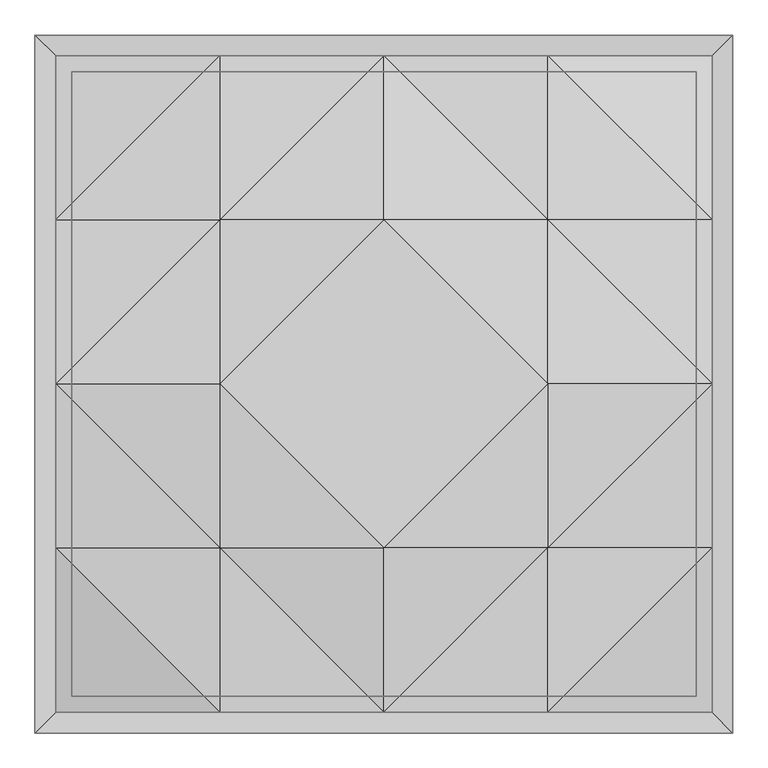
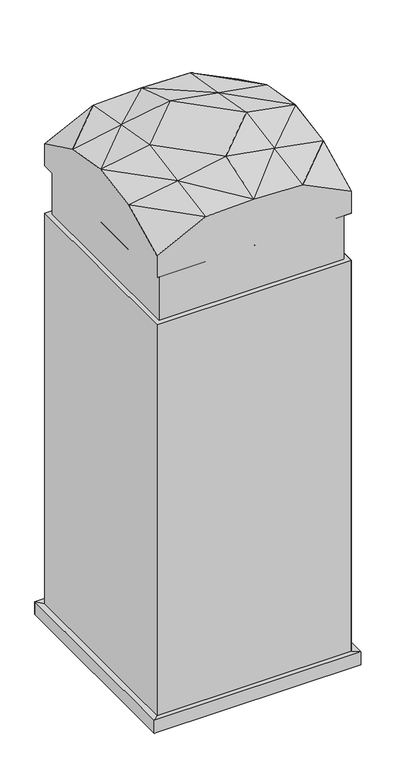
"""IFC4 building model written with IfcOpenShell, lengths in millimetres: geographic element geometry, Enscape AssetDefinition - Phonebooth 001 : Enscape AssetDefinition - Phonebooth 001."""

import ifcopenshell
import ifcopenshell.guid

model = None  # the IFC model being written
_history = None  # IfcOwnerHistory: only IFC2X3 demands one
_inside = {}  # id of a spatial element -> (the spatial element, [elements in it])
_under = {}  # id of a project, library or spatial element -> (it, [spatial elements below it])
_declared = {}  # id of a project -> (the project, [libraries it declares])
_typed = {}  # id of a type object -> (the type object, [elements of that type])
_made_of = {}  # id of a material, layer set ... -> (it, [elements and type objects made of it])


def new_model(schema):
    """Start an empty IFC model of exactly this schema.

    Asked for "IFC4X3", IfcOpenShell would pick the latest addendum, in which some entities
    have other attributes; the version numbers below select the first issue.
    IFC2X3 requires an IfcOwnerHistory on every rooted entity: one is made here for all.
    """
    global model, _history
    if schema == "IFC4X3":
        model = ifcopenshell.file(schema_version=(4, 3, 0, 0))
    else:
        model = ifcopenshell.file(schema=schema)
    _inside.clear()
    _under.clear()
    _declared.clear()
    _typed.clear()
    _made_of.clear()
    _history = None
    if model.schema == "IFC2X3":
        org = make("IfcOrganization", Name="unknown")
        user = make(
            "IfcPersonAndOrganization",
            ThePerson=make("IfcPerson", FamilyName="unknown"),
            TheOrganization=org,
        )
        app = make(
            "IfcApplication",
            ApplicationDeveloper=org,
            Version="unknown",
            ApplicationFullName="unknown",
            ApplicationIdentifier="unknown",
        )
        _history = make(
            "IfcOwnerHistory",
            OwningUser=user,
            OwningApplication=app,
            ChangeAction="ADDED",
            CreationDate=0,
        )
    return model


def make(cls, **values):
    """One entity of the class cls with the attributes given. An attribute that is None is left unset."""
    return model.create_entity(
        cls, **{name: value for name, value in values.items() if value is not None}
    )


def rooted(cls, **values):
    """An entity with a GlobalId (a new one), such as an element, a storey or a relation."""
    return make(cls, GlobalId=ifcopenshell.guid.new(), OwnerHistory=_history, **values)


def si_unit(unit_type, name, prefix=None):
    """IfcSIUnit, for example si_unit("LENGTHUNIT", "METRE", prefix="MILLI")."""
    return make("IfcSIUnit", UnitType=unit_type, Prefix=prefix, Name=name)


def assignment(units):
    """IfcUnitAssignment: the units of a project."""
    return None if units is None else make("IfcUnitAssignment", Units=units)


def point(xyz):
    """IfcCartesianPoint."""
    return None if xyz is None else make("IfcCartesianPoint", Coordinates=xyz)


def direction(xyz):
    """IfcDirection."""
    return None if xyz is None else make("IfcDirection", DirectionRatios=xyz)


def frame(location, z_axis=None, x_axis=None):
    """IfcAxis2Placement3D, a coordinate frame: its origin and axes. An axis left out is left unset."""
    return make(
        "IfcAxis2Placement3D",
        Location=point(location),
        Axis=direction(z_axis),
        RefDirection=direction(x_axis),
    )


def origin():
    """The frame at (0, 0, 0) with its axes left unset."""
    return frame((0.0, 0.0, 0.0))


def place(relative_to, where):
    """IfcLocalPlacement: puts the frame where relative to a parent placement (None: the world)."""
    return make(
        "IfcLocalPlacement", PlacementRelTo=relative_to, RelativePlacement=where
    )


def context(
    kind, dimensions, precision=None, world=None, true_north=None, identifier=None
):
    """IfcGeometricRepresentationContext, for example the 3D "Model" context."""
    return make(
        "IfcGeometricRepresentationContext",
        ContextIdentifier=identifier,
        ContextType=kind,
        CoordinateSpaceDimension=dimensions,
        Precision=precision,
        WorldCoordinateSystem=world,
        TrueNorth=true_north,
    )


def project(units=None, contexts=None):
    """IfcProject with its units and contexts."""
    return rooted(
        "IfcProject",
        Name="project",
        RepresentationContexts=contexts,
        UnitsInContext=assignment(units),
    )


def spatial(cls, under=None, at=None, **own):
    """A site, building, storey or space (cls), placed at a placement, below another one or the project."""
    s = rooted(cls, ObjectPlacement=at, **own)
    if under is not None:
        _under.setdefault(under.id(), (under, []))[1].append(s)
    return s


def point_list(points):
    """IfcCartesianPointList2D or 3D."""
    cls = (
        "IfcCartesianPointList2D" if len(points[0]) == 2 else "IfcCartesianPointList3D"
    )
    return make(cls, CoordList=points)


def triangles(points, corners, closed=None, point_numbers=None):
    """IfcTriangulatedFaceSet: each triangle names its three corners, points numbered from 1."""
    return make(
        "IfcTriangulatedFaceSet",
        Coordinates=point_list(points),
        Closed=closed,
        CoordIndex=corners,
        PnIndex=point_numbers,
    )


def shape(context_of_items, identifier, shape_type, items):
    """IfcShapeRepresentation: the items that make up one representation, for example the "Body"."""
    return make(
        "IfcShapeRepresentation",
        ContextOfItems=context_of_items,
        RepresentationIdentifier=identifier,
        RepresentationType=shape_type,
        Items=items,
    )


def source(mapping_origin, context_of_items, identifier, shape_type, items):
    """IfcRepresentationMap: a shape defined once, which mapped items show again and again."""
    return make(
        "IfcRepresentationMap",
        MappingOrigin=mapping_origin,
        MappedRepresentation=shape(context_of_items, identifier, shape_type, items),
    )


def transform(
    local_origin,
    x_axis=None,
    y_axis=None,
    z_axis=None,
    scale=None,
    scale2=None,
    scale3=None,
    uniform=True,
):
    """IfcCartesianTransformationOperator3D, or its non-uniform kind. x_axis, y_axis, z_axis: its Axis1, 2, 3."""
    if uniform:
        return make(
            "IfcCartesianTransformationOperator3D",
            Axis1=direction(x_axis),
            Axis2=direction(y_axis),
            LocalOrigin=point(local_origin),
            Scale=scale,
            Axis3=direction(z_axis),
        )
    return make(
        "IfcCartesianTransformationOperator3DnonUniform",
        Axis1=direction(x_axis),
        Axis2=direction(y_axis),
        LocalOrigin=point(local_origin),
        Scale=scale,
        Axis3=direction(z_axis),
        Scale2=scale2,
        Scale3=scale3,
    )


def mapped(mapping_source, mapping_target):
    """IfcMappedItem: shows the shape of a source again, moved by a transform."""
    return make(
        "IfcMappedItem", MappingSource=mapping_source, MappingTarget=mapping_target
    )


def made_of(thing, what):
    """Note that an element or type object is made of a material, layer set ...; save() writes the relation."""
    if what is not None:
        _made_of.setdefault(what.id(), (what, []))[1].append(thing)
    return thing


def element(
    cls,
    number,
    at=None,
    inside=None,
    cuts=None,
    type_object=None,
    material=None,
    context=None,
    identifier="Body",
    shape_type=None,
    held_by="IfcProductDefinitionShape",
    body=None,
    shapes=None,
    **own,
):
    """One element of the class cls, such as IfcWall. Its Tag is "e" and its number.

    at: its placement. inside: the storey or other place that contains it. cuts: it is an
    opening in that element (IfcRelVoidsElement). A single representation is given by context,
    identifier, shape_type and body (its items); several are given by shapes. held_by: the class
    of the entity that holds the representations. save() writes the other relations.
    """
    e = rooted(cls, Tag="e%d" % number, ObjectPlacement=at, **own)
    if body is not None:
        shapes = [shape(context, identifier, shape_type, body)]
    if shapes is not None:
        e.Representation = make(held_by, Representations=shapes)
    if inside is not None:
        _inside.setdefault(inside.id(), (inside, []))[1].append(e)
    if cuts is not None:
        rooted(
            "IfcRelVoidsElement", RelatingBuildingElement=cuts, RelatedOpeningElement=e
        )
    if type_object is not None:
        _typed.setdefault(type_object.id(), (type_object, []))[1].append(e)
    return made_of(e, material)


def aggregate(whole, parts):
    """IfcRelAggregates: a whole, such as a stair, and the parts it consists of."""
    return rooted("IfcRelAggregates", RelatingObject=whole, RelatedObjects=parts)


def save(model, path):
    """Write the relations noted so far, then the file.

    IfcRelAggregates (storeys below a building ...), IfcRelContainedInSpatialStructure (elements
    in a storey), IfcRelDefinesByType, IfcRelAssociatesMaterial and IfcRelDeclares: one each for
    every whole, place, type object, material and project.
    """
    for whole, parts in _under.values():
        aggregate(whole, parts)
    for where, things in _inside.values():
        rooted(
            "IfcRelContainedInSpatialStructure",
            RelatedElements=things,
            RelatingStructure=where,
        )
    for kind, things in _typed.values():
        rooted("IfcRelDefinesByType", RelatedObjects=things, RelatingType=kind)
    for what, things in _made_of.values():
        rooted("IfcRelAssociatesMaterial", RelatedObjects=things, RelatingMaterial=what)
    for by, libraries in _declared.values():
        rooted("IfcRelDeclares", RelatingContext=by, RelatedDefinitions=libraries)
    model.write(path)


def geographic_element_4e0d1d1e(model_context):
    return source(origin(), model_context, "Body", "Tessellation", [
        triangles([(535.4750187, 563.9070405, 65.5929985), (-535.4750187, -563.9070405, 65.5929985), (563.9070405, -563.9070405, 73.6019982), (-530.4179873, -530.4179873, 69.2310031), (-530.4179873, 530.4179873, 2320.0650719), (-563.9070405, -563.9070405, 73.6019982), (-530.4179873, -530.4179873, 2320.0650719), (-504.6510281, -504.6510281, 2320.0650719), (-504.6510281, -504.6510281, 2591.2188698), (-504.6510281, 504.6510281, 2320.0650719), (504.6510281, 504.6510281, 2320.0650719), (530.4179873, 530.4179873, 2320.0650719), (504.6510281, -504.6510281, 2320.0650719), (504.6510281, 504.6510281, 2591.2188698), (-530.4179873, 530.4179873, 69.2310031), (530.4179873, -530.4179873, 2320.0650719), (530.4179873, -530.4179873, 69.2310031), (530.4179873, 530.4179873, 69.2310031), (-563.9070405, 563.9070405, 73.6019982), (563.9070405, 563.9070405, 0.0), (-535.4750187, 563.9070405, 65.5929985), (-563.9070405, 563.9070405, 0.0), (-563.9070405, -563.9070405, 0.0), (535.4750187, -563.9070405, 65.5929985), (563.9070405, -563.9070405, 0.0), (563.9070405, 563.9070405, 73.6019982), (-530.4179873, 0.0, 2591.2188698), (0.0, -530.4179873, 2591.2188698), (530.4179873, -530.4179873, 2591.2188698), (504.6510281, -504.6510281, 2591.2188698), (0.0, 530.4179873, 2591.2188698), (-504.6510281, 504.6510281, 2591.2188698), (-265.2089936, 530.4179873, 2848.6720505), (530.4179873, 530.4179873, 2591.2188698), (265.2089936, 530.4179873, 2848.6720505), (530.4179873, 530.4179873, 2717.9288681), (530.4179873, 265.2089936, 2848.6720505), (0.0, 265.2089936, 2942.3451118), (0.0, 530.4179873, 2855.5079704), (-265.2089936, 265.2089936, 2895.5090172), (265.2089936, 0.0, 2942.3451118), (265.2089936, 265.2089936, 2895.5090172), (530.4179873, 0.0, 2892.5769287), (265.2089936, -265.2089936, 2895.5090172), (0.0, 0.0, 2942.3451118), (-265.2089936, 0.0, 2942.3451118), (0.0, -265.2089936, 2942.3451118), (0.0, -530.4179873, 2855.5079704), (-530.4179873, -265.2089936, 2848.6720505), (-265.2089936, -265.2089936, 2895.5090172), (-530.4179873, 0.0, 2892.5769287), (-530.4179873, 265.2089936, 2848.6720505), (-530.4179873, -530.4179873, 2717.9288681), (-530.4179873, -530.4179873, 2591.2188698), (-265.2089936, -530.4179873, 2848.6720505), (265.2089936, -530.4179873, 2848.6720505), (530.4179873, -265.2089936, 2848.6720505), (530.4179873, -530.4179873, 2717.9288681), (530.4179873, 0.0, 2591.2188698), (-530.4179873, 530.4179873, 2591.2188698), (-530.4179873, 530.4179873, 2717.9288681)], [[33, 52, 40], [33, 61, 52], [60, 61, 33], [60, 52, 61], [60, 27, 52], [57, 56, 58], [29, 59, 57], [29, 58, 56], [29, 57, 58], [29, 56, 28], [54, 28, 55], [54, 55, 53], [49, 53, 55], [54, 53, 49], [54, 49, 27], [40, 52, 51], [27, 49, 51], [27, 51, 52], [40, 51, 46], [51, 49, 50], [51, 50, 46], [49, 55, 50], [50, 55, 48], [28, 56, 48], [28, 48, 55], [57, 44, 56], [44, 48, 56], [46, 50, 47], [44, 47, 48], [50, 48, 47], [46, 47, 45], [38, 40, 46], [38, 46, 45], [41, 45, 47], [38, 45, 41], [41, 47, 44], [43, 41, 44], [43, 44, 57], [59, 43, 57], [59, 37, 43], [42, 41, 43], [42, 43, 37], [38, 41, 42], [39, 38, 42], [39, 33, 40], [39, 40, 38], [35, 42, 37], [39, 42, 35], [35, 37, 36], [34, 36, 37], [34, 35, 36], [34, 37, 59], [34, 31, 35], [31, 33, 39], [31, 39, 35], [60, 33, 31], [27, 60, 32], [32, 60, 31], [14, 34, 59], [31, 34, 14], [31, 14, 32], [59, 29, 30], [30, 29, 28], [59, 30, 14], [9, 54, 27], [28, 54, 9], [27, 32, 9], [28, 9, 30], [26, 1, 21], [26, 25, 20], [26, 3, 25], [26, 17, 3], [3, 23, 25], [6, 2, 24], [3, 6, 23], [6, 24, 3], [6, 22, 23], [6, 19, 22], [19, 26, 20], [26, 21, 19], [19, 20, 22], [6, 15, 19], [26, 18, 17], [19, 15, 18], [19, 18, 26], [18, 16, 17], [15, 5, 12], [18, 12, 16], [15, 12, 18], [13, 30, 9], [16, 12, 13], [11, 14, 30], [12, 11, 13], [11, 30, 13], [10, 32, 14], [12, 5, 10], [10, 14, 11], [12, 10, 11], [8, 9, 32], [16, 13, 8], [8, 32, 10], [13, 9, 8], [7, 8, 10], [5, 7, 10], [16, 8, 7], [4, 17, 16], [6, 4, 15], [3, 17, 4], [4, 7, 5], [4, 16, 7], [3, 4, 6], [4, 5, 15]], closed=False),
    ])


if __name__ == "__main__":
    model = new_model("IFC4")
    model_context = context("Model", 3, world=origin())
    ifc_project = project(units=[si_unit("LENGTHUNIT", "METRE", prefix="MILLI")], contexts=[model_context])
    site = spatial("IfcSite", under=ifc_project)
    building = spatial("IfcBuilding", under=site)
    placement = place(None, origin())
    geographic_element_shape = geographic_element_4e0d1d1e(model_context)
    element("IfcGeographicElement", 1, ObjectType="Enscape AssetDefinition - Phonebooth 001 : Enscape AssetDefinition - Phonebooth 001", at=placement, inside=building, context=model_context, shape_type="MappedRepresentation", body=[
        mapped(geographic_element_shape, transform((0.0, 0.0, 0.0), x_axis=(1.0, 0.0, 0.0), y_axis=(0.0, 1.0, 0.0), z_axis=(0.0, 0.0, 1.0))),
    ])
    save(model, "model.ifc")

# Revit data of these elements
# Type "Enscape AssetDefinition - Phonebooth 001 : Enscape AssetDefinition - Phonebooth 001"
#   EnscapeAssetSource = "REMOTE"
#   EnscapeAssetId = "cbaa4123-c8af-4927-a697-0b826d016a1a"
#   Height = 2.942345 m
#   EnscapeNativeAssetHeight = 2.942345 m
#   Default Elevation = 0
